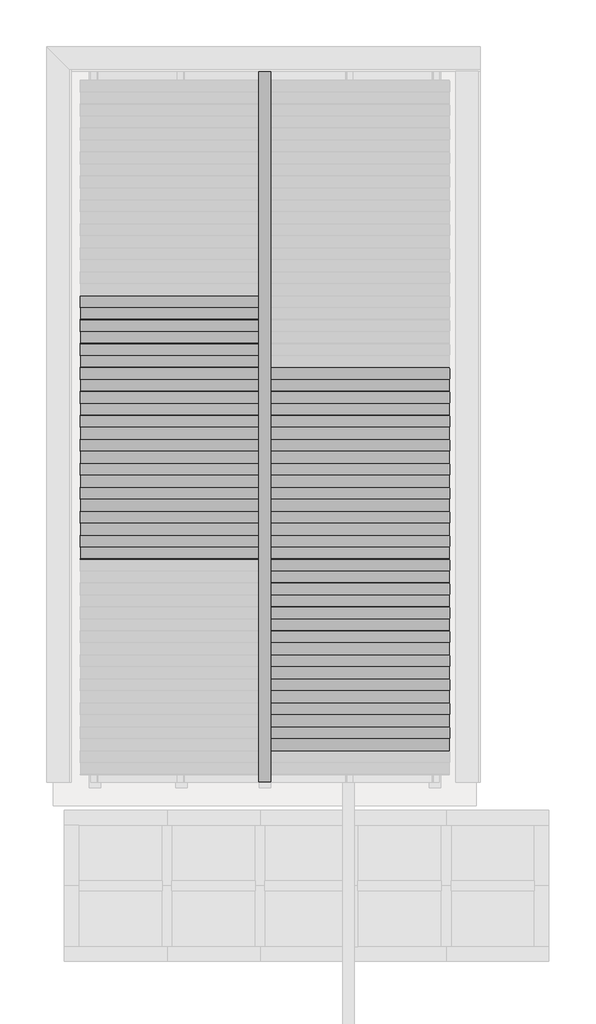
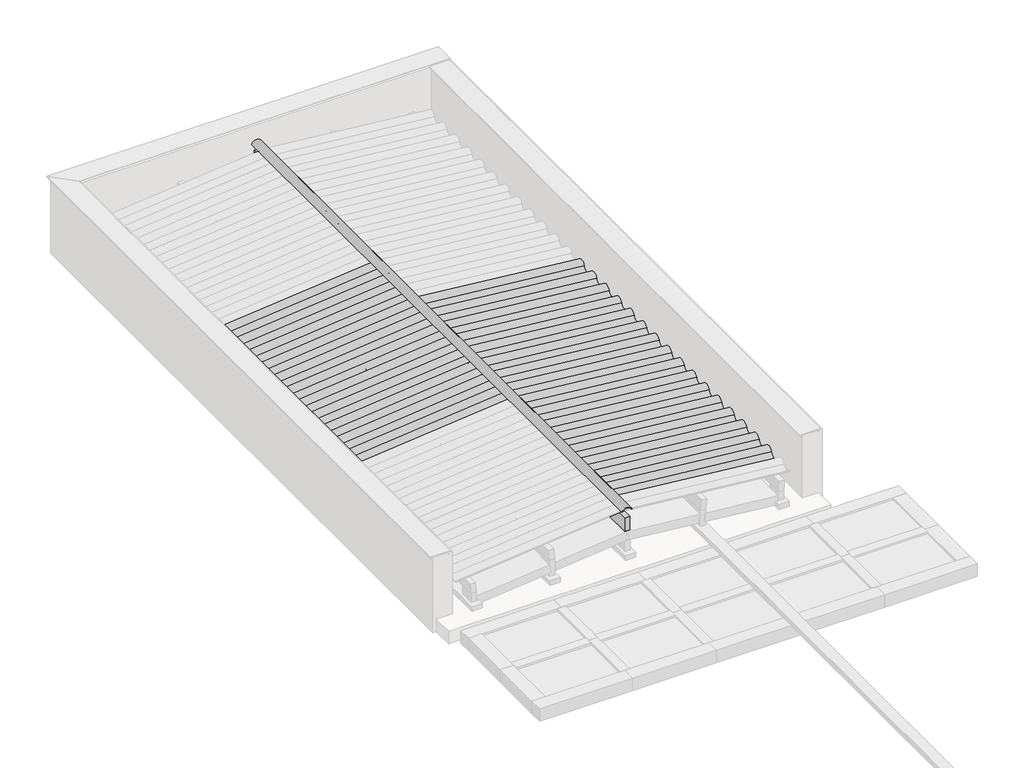
# One storey, part 2 of 3: 34 beams, 6 columns.
"""IFC4 building model written with IfcOpenShell, lengths in millimetres."""

import ifcopenshell
import ifcopenshell.guid

model = None  # the IFC model being written
_history = None  # IfcOwnerHistory: only IFC2X3 demands one
_inside = {}  # id of a spatial element -> (the spatial element, [elements in it])
_under = {}  # id of a project, library or spatial element -> (it, [spatial elements below it])
_declared = {}  # id of a project -> (the project, [libraries it declares])
_typed = {}  # id of a type object -> (the type object, [elements of that type])
_made_of = {}  # id of a material, layer set ... -> (it, [elements and type objects made of it])


def new_model(schema):
    """Start an empty IFC model of exactly this schema.

    Asked for "IFC4X3", IfcOpenShell would pick the latest addendum, in which some entities
    have other attributes; the version numbers below select the first issue.
    IFC2X3 requires an IfcOwnerHistory on every rooted entity: one is made here for all.
    """
    global model, _history
    if schema == "IFC4X3":
        model = ifcopenshell.file(schema_version=(4, 3, 0, 0))
    else:
        model = ifcopenshell.file(schema=schema)
    _inside.clear()
    _under.clear()
    _declared.clear()
    _typed.clear()
    _made_of.clear()
    _history = None
    if model.schema == "IFC2X3":
        org = make("IfcOrganization", Name="unknown")
        user = make(
            "IfcPersonAndOrganization",
            ThePerson=make("IfcPerson", FamilyName="unknown"),
            TheOrganization=org,
        )
        app = make(
            "IfcApplication",
            ApplicationDeveloper=org,
            Version="unknown",
            ApplicationFullName="unknown",
            ApplicationIdentifier="unknown",
        )
        _history = make(
            "IfcOwnerHistory",
            OwningUser=user,
            OwningApplication=app,
            ChangeAction="ADDED",
            CreationDate=0,
        )
    return model


def make(cls, **values):
    """One entity of the class cls with the attributes given. An attribute that is None is left unset."""
    return model.create_entity(
        cls, **{name: value for name, value in values.items() if value is not None}
    )


def rooted(cls, **values):
    """An entity with a GlobalId (a new one), such as an element, a storey or a relation."""
    return make(cls, GlobalId=ifcopenshell.guid.new(), OwnerHistory=_history, **values)


def si_unit(unit_type, name, prefix=None):
    """IfcSIUnit, for example si_unit("LENGTHUNIT", "METRE", prefix="MILLI")."""
    return make("IfcSIUnit", UnitType=unit_type, Prefix=prefix, Name=name)


def assignment(units):
    """IfcUnitAssignment: the units of a project."""
    return None if units is None else make("IfcUnitAssignment", Units=units)


def point(xyz):
    """IfcCartesianPoint."""
    return None if xyz is None else make("IfcCartesianPoint", Coordinates=xyz)


def direction(xyz):
    """IfcDirection."""
    return None if xyz is None else make("IfcDirection", DirectionRatios=xyz)


def frame(location, z_axis=None, x_axis=None):
    """IfcAxis2Placement3D, a coordinate frame: its origin and axes. An axis left out is left unset."""
    return make(
        "IfcAxis2Placement3D",
        Location=point(location),
        Axis=direction(z_axis),
        RefDirection=direction(x_axis),
    )


def frame_2d(location, x_axis=None):
    """IfcAxis2Placement2D, a coordinate frame in the plane: its origin and x axis."""
    return make(
        "IfcAxis2Placement2D", Location=point(location), RefDirection=direction(x_axis)
    )


def origin():
    """The frame at (0, 0, 0) with its axes left unset."""
    return frame((0.0, 0.0, 0.0))


def place(relative_to, where):
    """IfcLocalPlacement: puts the frame where relative to a parent placement (None: the world)."""
    return make(
        "IfcLocalPlacement", PlacementRelTo=relative_to, RelativePlacement=where
    )


def context(
    kind, dimensions, precision=None, world=None, true_north=None, identifier=None
):
    """IfcGeometricRepresentationContext, for example the 3D "Model" context."""
    return make(
        "IfcGeometricRepresentationContext",
        ContextIdentifier=identifier,
        ContextType=kind,
        CoordinateSpaceDimension=dimensions,
        Precision=precision,
        WorldCoordinateSystem=world,
        TrueNorth=true_north,
    )


def project(units=None, contexts=None):
    """IfcProject with its units and contexts."""
    return rooted(
        "IfcProject",
        Name="project",
        RepresentationContexts=contexts,
        UnitsInContext=assignment(units),
    )


def spatial(cls, under=None, at=None, **own):
    """A site, building, storey or space (cls), placed at a placement, below another one or the project."""
    s = rooted(cls, ObjectPlacement=at, **own)
    if under is not None:
        _under.setdefault(under.id(), (under, []))[1].append(s)
    return s


def polyline(points):
    """IfcPolyline through the points."""
    return make("IfcPolyline", Points=[point(p) for p in points])


def circle_curve(where, radius):
    """IfcCircle in the frame where."""
    return make("IfcCircle", Position=where, Radius=radius)


def trimmed(basis, trim1, trim2, sense, master):
    """IfcTrimmedCurve: the piece of a basis curve between two trims."""
    return make(
        "IfcTrimmedCurve",
        BasisCurve=basis,
        Trim1=trim1,
        Trim2=trim2,
        SenseAgreement=sense,
        MasterRepresentation=master,
    )


def segment(curve, same_sense, transition):
    """IfcCompositeCurveSegment."""
    return make(
        "IfcCompositeCurveSegment",
        Transition=transition,
        SameSense=same_sense,
        ParentCurve=curve,
    )


def composite_curve(segments, self_intersect=None):
    """IfcCompositeCurve: segments joined end to end."""
    return make("IfcCompositeCurve", Segments=segments, SelfIntersect=self_intersect)


def outline(outer, holes=None, kind="AREA"):
    """IfcArbitraryClosedProfileDef: a profile drawn as a closed curve; with holes, ...WithVoids."""
    if holes is None:
        return make("IfcArbitraryClosedProfileDef", ProfileType=kind, OuterCurve=outer)
    return make(
        "IfcArbitraryProfileDefWithVoids",
        ProfileType=kind,
        OuterCurve=outer,
        InnerCurves=holes,
    )


def extrude(swept, where, along, depth):
    """IfcExtrudedAreaSolid: the profile swept, set in the frame where, extruded along a direction by depth."""
    return make(
        "IfcExtrudedAreaSolid",
        SweptArea=swept,
        Position=where,
        ExtrudedDirection=direction(along),
        Depth=depth,
    )


def shape(context_of_items, identifier, shape_type, items):
    """IfcShapeRepresentation: the items that make up one representation, for example the "Body"."""
    return make(
        "IfcShapeRepresentation",
        ContextOfItems=context_of_items,
        RepresentationIdentifier=identifier,
        RepresentationType=shape_type,
        Items=items,
    )


def source(mapping_origin, context_of_items, identifier, shape_type, items):
    """IfcRepresentationMap: a shape defined once, which mapped items show again and again."""
    return make(
        "IfcRepresentationMap",
        MappingOrigin=mapping_origin,
        MappedRepresentation=shape(context_of_items, identifier, shape_type, items),
    )


def transform(
    local_origin,
    x_axis=None,
    y_axis=None,
    z_axis=None,
    scale=None,
    scale2=None,
    scale3=None,
    uniform=True,
):
    """IfcCartesianTransformationOperator3D, or its non-uniform kind. x_axis, y_axis, z_axis: its Axis1, 2, 3."""
    if uniform:
        return make(
            "IfcCartesianTransformationOperator3D",
            Axis1=direction(x_axis),
            Axis2=direction(y_axis),
            LocalOrigin=point(local_origin),
            Scale=scale,
            Axis3=direction(z_axis),
        )
    return make(
        "IfcCartesianTransformationOperator3DnonUniform",
        Axis1=direction(x_axis),
        Axis2=direction(y_axis),
        LocalOrigin=point(local_origin),
        Scale=scale,
        Axis3=direction(z_axis),
        Scale2=scale2,
        Scale3=scale3,
    )


def mapped(mapping_source, mapping_target):
    """IfcMappedItem: shows the shape of a source again, moved by a transform."""
    return make(
        "IfcMappedItem", MappingSource=mapping_source, MappingTarget=mapping_target
    )


def made_of(thing, what):
    """Note that an element or type object is made of a material, layer set ...; save() writes the relation."""
    if what is not None:
        _made_of.setdefault(what.id(), (what, []))[1].append(thing)
    return thing


def element(
    cls,
    number,
    at=None,
    inside=None,
    cuts=None,
    type_object=None,
    material=None,
    context=None,
    identifier="Body",
    shape_type=None,
    held_by="IfcProductDefinitionShape",
    body=None,
    shapes=None,
    **own,
):
    """One element of the class cls, such as IfcWall. Its Tag is "e" and its number.

    at: its placement. inside: the storey or other place that contains it. cuts: it is an
    opening in that element (IfcRelVoidsElement). A single representation is given by context,
    identifier, shape_type and body (its items); several are given by shapes. held_by: the class
    of the entity that holds the representations. save() writes the other relations.
    """
    e = rooted(cls, Tag="e%d" % number, ObjectPlacement=at, **own)
    if body is not None:
        shapes = [shape(context, identifier, shape_type, body)]
    if shapes is not None:
        e.Representation = make(held_by, Representations=shapes)
    if inside is not None:
        _inside.setdefault(inside.id(), (inside, []))[1].append(e)
    if cuts is not None:
        rooted(
            "IfcRelVoidsElement", RelatingBuildingElement=cuts, RelatedOpeningElement=e
        )
    if type_object is not None:
        _typed.setdefault(type_object.id(), (type_object, []))[1].append(e)
    return made_of(e, material)


def aggregate(whole, parts):
    """IfcRelAggregates: a whole, such as a stair, and the parts it consists of."""
    return rooted("IfcRelAggregates", RelatingObject=whole, RelatedObjects=parts)


def save(model, path):
    """Write the relations noted so far, then the file.

    IfcRelAggregates (storeys below a building ...), IfcRelContainedInSpatialStructure (elements
    in a storey), IfcRelDefinesByType, IfcRelAssociatesMaterial and IfcRelDeclares: one each for
    every whole, place, type object, material and project.
    """
    for whole, parts in _under.values():
        aggregate(whole, parts)
    for where, things in _inside.values():
        rooted(
            "IfcRelContainedInSpatialStructure",
            RelatedElements=things,
            RelatingStructure=where,
        )
    for kind, things in _typed.values():
        rooted("IfcRelDefinesByType", RelatedObjects=things, RelatingType=kind)
    for what, things in _made_of.values():
        rooted("IfcRelAssociatesMaterial", RelatedObjects=things, RelatingMaterial=what)
    for by, libraries in _declared.values():
        rooted("IfcRelDeclares", RelatingContext=by, RelatedDefinitions=libraries)
    model.write(path)


def cumeeira_telha_ondulada_fibrocimento_28917381(model_context):
    return source(origin(), model_context, "Body", "SweptSolid", [
        extrude(outline(composite_curve([segment(polyline([(58.3970135, 42.4437972), (53.9055884, 40.2467307)]), True, "CONTINUOUS"), segment(trimmed(circle_curve(frame_2d((-1.6029865, 13.0936483)), 61.7939461), [point((53.9055884, 40.2467307))], [point((-57.1115615, 40.2467307))], True, "CARTESIAN"), True, "CONTINUOUS"), segment(polyline([(-57.1115615, 40.2467307), (-61.6029865, 42.4437972)]), True, "CONTINUOUS"), segment(trimmed(circle_curve(frame_2d((-1.6029865, 13.0936483)), 66.7939461), [point((-61.6029865, 42.4437972))], [point((58.3970135, 42.4437972))], False, "CARTESIAN"), True, "CONTINUOUS")], self_intersect=False)), frame((-3626.5, 0.0, 0.0), z_axis=(1.0, 0.0, 0.0), x_axis=(0.0, 1.0, 0.0)), (0.0, 0.0, 1.0), 7253.0),
    ])


def viga_cumeeira_6x16cm_d80f05ee(model_context):
    return source(origin(), model_context, "Body", "SweptSolid", [
        extrude(outline(polyline([(3626.5, 30.0), (3626.5, -30.0), (-3626.5, -30.0), (-3626.5, 30.0), (3626.5, 30.0)])), frame((0.0, 0.0, -80.0), z_axis=(0.0, 0.0, 1.0), x_axis=(1.0, 0.0, 0.0)), (0.0, 0.0, 1.0), 160.0),
    ])


def column_1cffec27(model_context):
    return source(origin(), model_context, "Body", "SweptSolid", [
        extrude(outline(polyline([(30.0, 80.0), (30.0, -80.0), (-30.0, -80.0), (-30.0, 80.0), (30.0, 80.0)])), frame((0.0, 0.0, 3110.0), z_axis=(0.0, 0.0, 1.0), x_axis=(1.0, 0.0, 0.0)), (0.0, 0.0, 1.0), 238.0),
    ])


def column_35730ad5(model_context):
    return source(origin(), model_context, "Body", "SweptSolid", [
        extrude(outline(polyline([(30.0, 80.0), (30.0, -80.0), (-30.0, -80.0), (-30.0, 80.0), (30.0, 80.0)])), frame((0.0, 0.0, 3110.0), z_axis=(0.0, 0.0, 1.0), x_axis=(1.0, 0.0, 0.0)), (0.0, 0.0, 1.0), 197.9),
    ])


def column_00c463e4(model_context):
    return source(origin(), model_context, "Body", "SweptSolid", [
        extrude(outline(polyline([(30.0, 80.0), (30.0, -80.0), (-30.0, -80.0), (-30.0, 80.0), (30.0, 80.0)])), frame((0.0, 0.0, 3110.0), z_axis=(0.0, 0.0, 1.0), x_axis=(1.0, 0.0, 0.0)), (0.0, 0.0, 1.0), 109.8),
    ])


model = new_model("IFC4")

# Units and contexts
model_context = context("Model", 3, world=origin())
ifc_project = project(units=[si_unit("LENGTHUNIT", "METRE", prefix="MILLI")], contexts=[model_context])

# Site, building, storey
site = spatial("IfcSite", under=ifc_project)
building = spatial("IfcBuilding", under=site)
storey = spatial("IfcBuildingStorey", under=building, Name="COB. GARAGEM", Elevation=3050.0)

# Beams
placement = place(None, origin())
element("IfcBeam", 1, ObjectType="Madeira de lei : Berço 6x12cm", at=placement, inside=storey, context=model_context, shape_type="SweptSolid", body=[
    extrude(outline(polyline([(-9620.281307, 4423.9300153), (-9500.281307, 4423.9300153), (-9500.281307, 2423.9300153), (-9620.281307, 2423.9300153), (-9620.281307, 4423.9300153)])), frame((0.0, 0.0, 3050.0), z_axis=(0.0, 0.0, 1.0), x_axis=(1.0, 0.0, 0.0)), (0.0, 0.0, 1.0), 60.0),
])
element("IfcBeam", 2, ObjectType="Madeira de lei : Berço 6x12cm", at=placement, inside=storey, context=model_context, shape_type="SweptSolid", body=[
    extrude(outline(polyline([(-9620.281307, 2423.9300153), (-9500.281307, 2423.9300153), (-9500.281307, 423.9300153), (-9620.281307, 423.9300153), (-9620.281307, 2423.9300153)])), frame((0.0, 0.0, 3050.0), z_axis=(0.0, 0.0, 1.0), x_axis=(1.0, 0.0, 0.0)), (0.0, 0.0, 1.0), 60.0),
])
element("IfcBeam", 3, ObjectType="Madeira de lei : Berço 6x12cm", at=placement, inside=storey, context=model_context, shape_type="SweptSolid", body=[
    extrude(outline(polyline([(-8767.0824227, 4423.9300153), (-8647.0824227, 4423.9300153), (-8647.0824227, 2423.9300153), (-8767.0824227, 2423.9300153), (-8767.0824227, 4423.9300153)])), frame((0.0, 0.0, 3050.0), z_axis=(0.0, 0.0, 1.0), x_axis=(1.0, 0.0, 0.0)), (0.0, 0.0, 1.0), 60.0),
])
element("IfcBeam", 4, ObjectType="Madeira de lei : Berço 6x12cm", at=placement, inside=storey, context=model_context, shape_type="SweptSolid", body=[
    extrude(outline(polyline([(-10473.4801913, 4423.9300153), (-10353.4801913, 4423.9300153), (-10353.4801913, 2423.9300153), (-10473.4801913, 2423.9300153), (-10473.4801913, 4423.9300153)])), frame((0.0, 0.0, 3050.0), z_axis=(0.0, 0.0, 1.0), x_axis=(1.0, 0.0, 0.0)), (0.0, 0.0, 1.0), 60.0),
])
element("IfcBeam", 5, ObjectType="Madeira de lei : Berço 6x12cm", at=placement, inside=storey, context=model_context, shape_type="SweptSolid", body=[
    extrude(outline(polyline([(-11356.5301913, 4423.9300153), (-11236.5301913, 4423.9300153), (-11236.5301913, 2423.9300153), (-11356.5301913, 2423.9300153), (-11356.5301913, 4423.9300153)])), frame((0.0, 0.0, 3050.0), z_axis=(0.0, 0.0, 1.0), x_axis=(1.0, 0.0, 0.0)), (0.0, 0.0, 1.0), 60.0),
])
cumeeira_telha_ondulada_fibrocimento_shape = cumeeira_telha_ondulada_fibrocimento_28917381(model_context)
element("IfcBeam", 6, ObjectType="Cumeeira Telha Ondulada : Fibrocimento", at=placement, inside=storey, context=model_context, shape_type="MappedRepresentation", body=[
    mapped(cumeeira_telha_ondulada_fibrocimento_shape, transform((-9560.281307, 3455.9300153, 3545.9751229), x_axis=(0.0, -1.0, 0.0), y_axis=(1.0, 0.0, 0.0), z_axis=(0.0, 0.0, 1.0))),
])
element("IfcBeam", 7, ObjectType="Telha Ondulada : Fibrocimento", at=placement, inside=storey, context=model_context, shape_type="SweptSolid", body=[
    extrude(outline(composite_curve([segment(trimmed(circle_curve(frame_2d((-58.7002979, -53.2060538)), 66.7939461), [point((-29.350149, 6.7939462))], [point((-29.350149, -113.2060538))], False, "CARTESIAN"), True, "CONTINUOUS"), segment(polyline([(-29.350149, -113.2060538), (-31.5472155, -108.7146288)]), True, "CONTINUOUS"), segment(trimmed(circle_curve(frame_2d((-58.7002979, -53.2060538)), 61.7939461), [point((-31.5472155, -108.7146288))], [point((-31.5472155, 2.3025211))], True, "CARTESIAN"), True, "CONTINUOUS"), segment(trimmed(circle_curve(frame_2d((0.0, 66.7939462)), 71.7939461), [point((-31.5472155, 2.3025211))], [point((-31.5472155, 131.2853712))], False, "CARTESIAN"), True, "CONTINUOUS"), segment(polyline([(-31.5472155, 131.2853712), (-29.350149, 126.7939462)]), True, "CONTINUOUS"), segment(trimmed(circle_curve(frame_2d((0.0, 66.7939462)), 66.7939461), [point((-29.350149, 126.7939462))], [point((-29.350149, 6.7939462))], True, "CARTESIAN"), True, "CONTINUOUS")], self_intersect=False)), frame((-11446.918865, 2229.326948, 3394.3067746), z_axis=(0.9950371902099892, 0.0, 0.09950371902099919), x_axis=(-0.09950371902099919, 0.0, 0.9950371902099892)), (0.0, 0.0, 1.0), 1886.8678854),
])
element("IfcBeam", 8, ObjectType="Telha Ondulada : Fibrocimento", at=placement, inside=storey, context=model_context, shape_type="SweptSolid", body=[
    extrude(outline(composite_curve([segment(trimmed(circle_curve(frame_2d((-58.7002979, -53.2060538)), 66.7939461), [point((-29.350149, 6.7939462))], [point((-29.350149, -113.2060538))], False, "CARTESIAN"), True, "CONTINUOUS"), segment(polyline([(-29.350149, -113.2060538), (-31.5472155, -108.7146288)]), True, "CONTINUOUS"), segment(trimmed(circle_curve(frame_2d((-58.7002979, -53.2060538)), 61.7939461), [point((-31.5472155, -108.7146288))], [point((-31.5472155, 2.3025211))], True, "CARTESIAN"), True, "CONTINUOUS"), segment(trimmed(circle_curve(frame_2d((0.0, 66.7939462)), 71.7939461), [point((-31.5472155, 2.3025211))], [point((-31.5472155, 131.2853712))], False, "CARTESIAN"), True, "CONTINUOUS"), segment(polyline([(-31.5472155, 131.2853712), (-29.350149, 126.7939462)]), True, "CONTINUOUS"), segment(trimmed(circle_curve(frame_2d((0.0, 66.7939462)), 66.7939461), [point((-29.350149, 126.7939462))], [point((-29.350149, 6.7939462))], True, "CARTESIAN"), True, "CONTINUOUS")], self_intersect=False)), frame((-11446.918865, 2473.826948, 3394.3067746), z_axis=(0.9950371902099892, 0.0, 0.09950371902099932), x_axis=(-0.09950371902099932, 0.0, 0.9950371902099892)), (0.0, 0.0, 1.0), 1886.8678854),
])
element("IfcBeam", 9, ObjectType="Telha Ondulada : Fibrocimento", at=placement, inside=storey, context=model_context, shape_type="SweptSolid", body=[
    extrude(outline(composite_curve([segment(trimmed(circle_curve(frame_2d((-58.7002979, -53.2060538)), 66.7939461), [point((-29.350149, 6.7939462))], [point((-29.350149, -113.2060538))], False, "CARTESIAN"), True, "CONTINUOUS"), segment(polyline([(-29.350149, -113.2060538), (-31.5472155, -108.7146288)]), True, "CONTINUOUS"), segment(trimmed(circle_curve(frame_2d((-58.7002979, -53.2060538)), 61.7939461), [point((-31.5472155, -108.7146288))], [point((-31.5472155, 2.3025211))], True, "CARTESIAN"), True, "CONTINUOUS"), segment(trimmed(circle_curve(frame_2d((0.0, 66.7939462)), 71.7939461), [point((-31.5472155, 2.3025211))], [point((-31.5472155, 131.2853712))], False, "CARTESIAN"), True, "CONTINUOUS"), segment(polyline([(-31.5472155, 131.2853712), (-29.350149, 126.7939462)]), True, "CONTINUOUS"), segment(trimmed(circle_curve(frame_2d((0.0, 66.7939462)), 66.7939461), [point((-29.350149, 126.7939462))], [point((-29.350149, 6.7939462))], True, "CARTESIAN"), True, "CONTINUOUS")], self_intersect=False)), frame((-11446.918865, 2718.326948, 3394.3067746), z_axis=(0.9950371902099892, 0.0, 0.09950371902099937), x_axis=(-0.09950371902099937, 0.0, 0.9950371902099892)), (0.0, 0.0, 1.0), 1886.8678854),
])
element("IfcBeam", 10, ObjectType="Telha Ondulada : Fibrocimento", at=placement, inside=storey, context=model_context, shape_type="SweptSolid", body=[
    extrude(outline(composite_curve([segment(trimmed(circle_curve(frame_2d((-58.7002979, -53.2060538)), 66.7939461), [point((-29.350149, 6.7939462))], [point((-29.350149, -113.2060538))], False, "CARTESIAN"), True, "CONTINUOUS"), segment(polyline([(-29.350149, -113.2060538), (-31.5472155, -108.7146288)]), True, "CONTINUOUS"), segment(trimmed(circle_curve(frame_2d((-58.7002979, -53.2060538)), 61.7939461), [point((-31.5472155, -108.7146288))], [point((-31.5472155, 2.3025211))], True, "CARTESIAN"), True, "CONTINUOUS"), segment(trimmed(circle_curve(frame_2d((0.0, 66.7939462)), 71.7939461), [point((-31.5472155, 2.3025211))], [point((-31.5472155, 131.2853712))], False, "CARTESIAN"), True, "CONTINUOUS"), segment(polyline([(-31.5472155, 131.2853712), (-29.350149, 126.7939462)]), True, "CONTINUOUS"), segment(trimmed(circle_curve(frame_2d((0.0, 66.7939462)), 66.7939461), [point((-29.350149, 126.7939462))], [point((-29.350149, 6.7939462))], True, "CARTESIAN"), True, "CONTINUOUS")], self_intersect=False)), frame((-11446.918865, 2962.826948, 3394.3067746), z_axis=(0.9950371902099892, 0.0, 0.09950371902099943), x_axis=(-0.09950371902099943, 0.0, 0.9950371902099892)), (0.0, 0.0, 1.0), 1886.8678854),
])
element("IfcBeam", 11, ObjectType="Telha Ondulada : Fibrocimento", at=placement, inside=storey, context=model_context, shape_type="SweptSolid", body=[
    extrude(outline(composite_curve([segment(trimmed(circle_curve(frame_2d((-58.7002979, -53.2060538)), 66.7939461), [point((-29.350149, 6.7939462))], [point((-29.350149, -113.2060538))], False, "CARTESIAN"), True, "CONTINUOUS"), segment(polyline([(-29.350149, -113.2060538), (-31.5472155, -108.7146288)]), True, "CONTINUOUS"), segment(trimmed(circle_curve(frame_2d((-58.7002979, -53.2060538)), 61.7939461), [point((-31.5472155, -108.7146288))], [point((-31.5472155, 2.3025211))], True, "CARTESIAN"), True, "CONTINUOUS"), segment(trimmed(circle_curve(frame_2d((0.0, 66.7939462)), 71.7939461), [point((-31.5472155, 2.3025211))], [point((-31.5472155, 131.2853712))], False, "CARTESIAN"), True, "CONTINUOUS"), segment(polyline([(-31.5472155, 131.2853712), (-29.350149, 126.7939462)]), True, "CONTINUOUS"), segment(trimmed(circle_curve(frame_2d((0.0, 66.7939462)), 66.7939461), [point((-29.350149, 126.7939462))], [point((-29.350149, 6.7939462))], True, "CARTESIAN"), True, "CONTINUOUS")], self_intersect=False)), frame((-11446.918865, 3207.326948, 3394.3067746), z_axis=(0.9950371902099892, 0.0, 0.09950371902099954), x_axis=(-0.09950371902099954, 0.0, 0.9950371902099892)), (0.0, 0.0, 1.0), 1886.8678854),
])
element("IfcBeam", 12, ObjectType="Telha Ondulada : Fibrocimento", at=placement, inside=storey, context=model_context, shape_type="SweptSolid", body=[
    extrude(outline(composite_curve([segment(trimmed(circle_curve(frame_2d((-58.7002979, -53.2060538)), 66.7939461), [point((-29.350149, 6.7939462))], [point((-29.350149, -113.2060538))], False, "CARTESIAN"), True, "CONTINUOUS"), segment(polyline([(-29.350149, -113.2060538), (-31.5472155, -108.7146288)]), True, "CONTINUOUS"), segment(trimmed(circle_curve(frame_2d((-58.7002979, -53.2060538)), 61.7939461), [point((-31.5472155, -108.7146288))], [point((-31.5472155, 2.3025211))], True, "CARTESIAN"), True, "CONTINUOUS"), segment(trimmed(circle_curve(frame_2d((0.0, 66.7939462)), 71.7939461), [point((-31.5472155, 2.3025211))], [point((-31.5472155, 131.2853712))], False, "CARTESIAN"), True, "CONTINUOUS"), segment(polyline([(-31.5472155, 131.2853712), (-29.350149, 126.7939462)]), True, "CONTINUOUS"), segment(trimmed(circle_curve(frame_2d((0.0, 66.7939462)), 66.7939461), [point((-29.350149, 126.7939462))], [point((-29.350149, 6.7939462))], True, "CARTESIAN"), True, "CONTINUOUS")], self_intersect=False)), frame((-11446.918865, 3451.826948, 3394.3067746), z_axis=(0.9950371902099892, 0.0, 0.09950371902099937), x_axis=(-0.09950371902099937, 0.0, 0.9950371902099892)), (0.0, 0.0, 1.0), 1886.8678854),
])
element("IfcBeam", 13, ObjectType="Telha Ondulada : Fibrocimento", at=placement, inside=storey, context=model_context, shape_type="SweptSolid", body=[
    extrude(outline(composite_curve([segment(trimmed(circle_curve(frame_2d((-58.7002979, -53.2060538)), 66.7939461), [point((-29.350149, 6.7939462))], [point((-29.350149, -113.2060538))], False, "CARTESIAN"), True, "CONTINUOUS"), segment(polyline([(-29.350149, -113.2060538), (-31.5472155, -108.7146288)]), True, "CONTINUOUS"), segment(trimmed(circle_curve(frame_2d((-58.7002979, -53.2060538)), 61.7939461), [point((-31.5472155, -108.7146288))], [point((-31.5472155, 2.3025211))], True, "CARTESIAN"), True, "CONTINUOUS"), segment(trimmed(circle_curve(frame_2d((0.0, 66.7939462)), 71.7939461), [point((-31.5472155, 2.3025211))], [point((-31.5472155, 131.2853712))], False, "CARTESIAN"), True, "CONTINUOUS"), segment(polyline([(-31.5472155, 131.2853712), (-29.350149, 126.7939462)]), True, "CONTINUOUS"), segment(trimmed(circle_curve(frame_2d((0.0, 66.7939462)), 66.7939461), [point((-29.350149, 126.7939462))], [point((-29.350149, 6.7939462))], True, "CARTESIAN"), True, "CONTINUOUS")], self_intersect=False)), frame((-11446.918865, 3696.326948, 3394.3067746), z_axis=(0.9950371902099892, 0.0, 0.09950371902099914), x_axis=(-0.09950371902099914, 0.0, 0.9950371902099892)), (0.0, 0.0, 1.0), 1886.8678854),
])
element("IfcBeam", 14, ObjectType="Telha Ondulada : Fibrocimento", at=placement, inside=storey, context=model_context, shape_type="SweptSolid", body=[
    extrude(outline(composite_curve([segment(trimmed(circle_curve(frame_2d((-58.7002979, -53.2060538)), 66.7939461), [point((-29.350149, 6.7939462))], [point((-29.350149, -113.2060538))], False, "CARTESIAN"), True, "CONTINUOUS"), segment(polyline([(-29.350149, -113.2060538), (-31.5472155, -108.7146288)]), True, "CONTINUOUS"), segment(trimmed(circle_curve(frame_2d((-58.7002979, -53.2060538)), 61.7939461), [point((-31.5472155, -108.7146288))], [point((-31.5472155, 2.3025211))], True, "CARTESIAN"), True, "CONTINUOUS"), segment(trimmed(circle_curve(frame_2d((0.0, 66.7939462)), 71.7939461), [point((-31.5472155, 2.3025211))], [point((-31.5472155, 131.2853712))], False, "CARTESIAN"), True, "CONTINUOUS"), segment(polyline([(-31.5472155, 131.2853712), (-29.350149, 126.7939462)]), True, "CONTINUOUS"), segment(trimmed(circle_curve(frame_2d((0.0, 66.7939462)), 66.7939461), [point((-29.350149, 126.7939462))], [point((-29.350149, 6.7939462))], True, "CARTESIAN"), True, "CONTINUOUS")], self_intersect=False)), frame((-11446.918865, 3940.826948, 3394.3067746), z_axis=(0.9950371902099892, 0.0, 0.09950371902099948), x_axis=(-0.09950371902099948, 0.0, 0.9950371902099892)), (0.0, 0.0, 1.0), 1886.8678854),
])
element("IfcBeam", 15, ObjectType="Telha Ondulada : Fibrocimento", at=placement, inside=storey, context=model_context, shape_type="SweptSolid", body=[
    extrude(outline(composite_curve([segment(trimmed(circle_curve(frame_2d((-58.7002979, -53.2060538)), 66.7939461), [point((-29.350149, 6.7939462))], [point((-29.350149, -113.2060538))], False, "CARTESIAN"), True, "CONTINUOUS"), segment(polyline([(-29.350149, -113.2060538), (-31.5472155, -108.7146288)]), True, "CONTINUOUS"), segment(trimmed(circle_curve(frame_2d((-58.7002979, -53.2060538)), 61.7939461), [point((-31.5472155, -108.7146288))], [point((-31.5472155, 2.3025211))], True, "CARTESIAN"), True, "CONTINUOUS"), segment(trimmed(circle_curve(frame_2d((0.0, 66.7939462)), 71.7939461), [point((-31.5472155, 2.3025211))], [point((-31.5472155, 131.2853712))], False, "CARTESIAN"), True, "CONTINUOUS"), segment(polyline([(-31.5472155, 131.2853712), (-29.350149, 126.7939462)]), True, "CONTINUOUS"), segment(trimmed(circle_curve(frame_2d((0.0, 66.7939462)), 66.7939461), [point((-29.350149, 126.7939462))], [point((-29.350149, 6.7939462))], True, "CARTESIAN"), True, "CONTINUOUS")], self_intersect=False)), frame((-11446.918865, 4185.326948, 3394.3067746), z_axis=(0.9950371902099892, 0.0, 0.09950371902099932), x_axis=(-0.09950371902099932, 0.0, 0.9950371902099892)), (0.0, 0.0, 1.0), 1886.8678854),
])
element("IfcBeam", 16, ObjectType="Telha Ondulada : Fibrocimento", at=placement, inside=storey, context=model_context, shape_type="SweptSolid", body=[
    extrude(outline(composite_curve([segment(trimmed(circle_curve(frame_2d((-58.7002979, -53.2060538)), 66.7939461), [point((-29.350149, 6.7939462))], [point((-29.350149, -113.2060538))], False, "CARTESIAN"), True, "CONTINUOUS"), segment(polyline([(-29.350149, -113.2060538), (-31.5472155, -108.7146288)]), True, "CONTINUOUS"), segment(trimmed(circle_curve(frame_2d((-58.7002979, -53.2060538)), 61.7939461), [point((-31.5472155, -108.7146288))], [point((-31.5472155, 2.3025211))], True, "CARTESIAN"), True, "CONTINUOUS"), segment(trimmed(circle_curve(frame_2d((0.0, 66.7939462)), 71.7939461), [point((-31.5472155, 2.3025211))], [point((-31.5472155, 131.2853712))], False, "CARTESIAN"), True, "CONTINUOUS"), segment(polyline([(-31.5472155, 131.2853712), (-29.350149, 126.7939462)]), True, "CONTINUOUS"), segment(trimmed(circle_curve(frame_2d((0.0, 66.7939462)), 66.7939461), [point((-29.350149, 126.7939462))], [point((-29.350149, 6.7939462))], True, "CARTESIAN"), True, "CONTINUOUS")], self_intersect=False)), frame((-11446.918865, 4429.826948, 3394.3067746), z_axis=(0.9950371902099892, 0.0, 0.09950371902099943), x_axis=(-0.09950371902099943, 0.0, 0.9950371902099892)), (0.0, 0.0, 1.0), 1886.8678854),
])
element("IfcBeam", 17, ObjectType="Telha Ondulada : Fibrocimento", at=placement, inside=storey, context=model_context, shape_type="SweptSolid", body=[
    extrude(outline(composite_curve([segment(trimmed(circle_curve(frame_2d((-58.7002979, -53.2060538)), 66.7939461), [point((-29.350149, 6.7939462))], [point((-29.350149, -113.2060538))], False, "CARTESIAN"), True, "CONTINUOUS"), segment(polyline([(-29.350149, -113.2060538), (-31.5472155, -108.7146288)]), True, "CONTINUOUS"), segment(trimmed(circle_curve(frame_2d((-58.7002979, -53.2060538)), 61.7939461), [point((-31.5472155, -108.7146288))], [point((-31.5472155, 2.3025211))], True, "CARTESIAN"), True, "CONTINUOUS"), segment(trimmed(circle_curve(frame_2d((0.0, 66.7939462)), 71.7939461), [point((-31.5472155, 2.3025211))], [point((-31.5472155, 131.2853712))], False, "CARTESIAN"), True, "CONTINUOUS"), segment(polyline([(-31.5472155, 131.2853712), (-29.350149, 126.7939462)]), True, "CONTINUOUS"), segment(trimmed(circle_curve(frame_2d((0.0, 66.7939462)), 66.7939461), [point((-29.350149, 126.7939462))], [point((-29.350149, 6.7939462))], True, "CARTESIAN"), True, "CONTINUOUS")], self_intersect=False)), frame((-11446.918865, 4674.326948, 3394.3067746), z_axis=(0.9950371902099892, 0.0, 0.09950371902099943), x_axis=(-0.09950371902099943, 0.0, 0.9950371902099892)), (0.0, 0.0, 1.0), 1886.8678854),
])
element("IfcBeam", 18, ObjectType="Telha Ondulada : Fibrocimento", at=placement, inside=storey, context=model_context, shape_type="SweptSolid", body=[
    extrude(outline(composite_curve([segment(trimmed(circle_curve(frame_2d((0.0, 66.7939462)), 66.7939461), [point((29.350149, 6.7939462))], [point((29.350149, 126.7939462))], True, "CARTESIAN"), True, "CONTINUOUS"), segment(polyline([(29.350149, 126.7939462), (31.5472155, 131.2853712)]), True, "CONTINUOUS"), segment(trimmed(circle_curve(frame_2d((0.0, 66.7939462)), 71.7939461), [point((31.5472155, 131.2853712))], [point((31.5472155, 2.3025211))], False, "CARTESIAN"), True, "CONTINUOUS"), segment(trimmed(circle_curve(frame_2d((58.7002979, -53.2060538)), 61.7939461), [point((31.5472155, 2.3025211))], [point((31.5472155, -108.7146288))], True, "CARTESIAN"), True, "CONTINUOUS"), segment(polyline([(31.5472155, -108.7146288), (29.350149, -113.2060538)]), True, "CONTINUOUS"), segment(trimmed(circle_curve(frame_2d((58.7002979, -53.2060538)), 66.7939461), [point((29.350149, -113.2060538))], [point((29.350149, 6.7939462))], False, "CARTESIAN"), True, "CONTINUOUS")], self_intersect=False)), frame((-7673.6437489, 273.326948, 3394.3067746), z_axis=(-0.9950371902099892, 0.0, 0.09950371902099979), x_axis=(-0.09950371902099979, 0.0, -0.9950371902099892)), (0.0, 0.0, 1.0), 1886.8678854),
])
element("IfcBeam", 19, ObjectType="Telha Ondulada : Fibrocimento", at=placement, inside=storey, context=model_context, shape_type="SweptSolid", body=[
    extrude(outline(composite_curve([segment(trimmed(circle_curve(frame_2d((0.0, 66.7939462)), 66.7939461), [point((29.350149, 6.7939462))], [point((29.350149, 126.7939462))], True, "CARTESIAN"), True, "CONTINUOUS"), segment(polyline([(29.350149, 126.7939462), (31.5472155, 131.2853712)]), True, "CONTINUOUS"), segment(trimmed(circle_curve(frame_2d((0.0, 66.7939462)), 71.7939461), [point((31.5472155, 131.2853712))], [point((31.5472155, 2.3025211))], False, "CARTESIAN"), True, "CONTINUOUS"), segment(trimmed(circle_curve(frame_2d((58.7002979, -53.2060538)), 61.7939461), [point((31.5472155, 2.3025211))], [point((31.5472155, -108.7146288))], True, "CARTESIAN"), True, "CONTINUOUS"), segment(polyline([(31.5472155, -108.7146288), (29.350149, -113.2060538)]), True, "CONTINUOUS"), segment(trimmed(circle_curve(frame_2d((58.7002979, -53.2060538)), 66.7939461), [point((29.350149, -113.2060538))], [point((29.350149, 6.7939462))], False, "CARTESIAN"), True, "CONTINUOUS")], self_intersect=False)), frame((-7673.6437489, 517.826948, 3394.3067746), z_axis=(-0.9950371902099892, 0.0, 0.09950371902099979), x_axis=(-0.09950371902099979, 0.0, -0.9950371902099892)), (0.0, 0.0, 1.0), 1886.8678854),
])
element("IfcBeam", 20, ObjectType="Telha Ondulada : Fibrocimento", at=placement, inside=storey, context=model_context, shape_type="SweptSolid", body=[
    extrude(outline(composite_curve([segment(trimmed(circle_curve(frame_2d((0.0, 66.7939462)), 66.7939461), [point((29.350149, 6.7939462))], [point((29.350149, 126.7939462))], True, "CARTESIAN"), True, "CONTINUOUS"), segment(polyline([(29.350149, 126.7939462), (31.5472155, 131.2853712)]), True, "CONTINUOUS"), segment(trimmed(circle_curve(frame_2d((0.0, 66.7939462)), 71.7939461), [point((31.5472155, 131.2853712))], [point((31.5472155, 2.3025211))], False, "CARTESIAN"), True, "CONTINUOUS"), segment(trimmed(circle_curve(frame_2d((58.7002979, -53.2060538)), 61.7939461), [point((31.5472155, 2.3025211))], [point((31.5472155, -108.7146288))], True, "CARTESIAN"), True, "CONTINUOUS"), segment(polyline([(31.5472155, -108.7146288), (29.350149, -113.2060538)]), True, "CONTINUOUS"), segment(trimmed(circle_curve(frame_2d((58.7002979, -53.2060538)), 66.7939461), [point((29.350149, -113.2060538))], [point((29.350149, 6.7939462))], False, "CARTESIAN"), True, "CONTINUOUS")], self_intersect=False)), frame((-7673.6437489, 762.326948, 3394.3067746), z_axis=(-0.9950371902099892, 0.0, 0.09950371902099979), x_axis=(-0.09950371902099979, 0.0, -0.9950371902099892)), (0.0, 0.0, 1.0), 1886.8678854),
])
element("IfcBeam", 21, ObjectType="Telha Ondulada : Fibrocimento", at=placement, inside=storey, context=model_context, shape_type="SweptSolid", body=[
    extrude(outline(composite_curve([segment(trimmed(circle_curve(frame_2d((0.0, 66.7939462)), 66.7939461), [point((29.350149, 6.7939462))], [point((29.350149, 126.7939462))], True, "CARTESIAN"), True, "CONTINUOUS"), segment(polyline([(29.350149, 126.7939462), (31.5472155, 131.2853712)]), True, "CONTINUOUS"), segment(trimmed(circle_curve(frame_2d((0.0, 66.7939462)), 71.7939461), [point((31.5472155, 131.2853712))], [point((31.5472155, 2.3025211))], False, "CARTESIAN"), True, "CONTINUOUS"), segment(trimmed(circle_curve(frame_2d((58.7002979, -53.2060538)), 61.7939461), [point((31.5472155, 2.3025211))], [point((31.5472155, -108.7146288))], True, "CARTESIAN"), True, "CONTINUOUS"), segment(polyline([(31.5472155, -108.7146288), (29.350149, -113.2060538)]), True, "CONTINUOUS"), segment(trimmed(circle_curve(frame_2d((58.7002979, -53.2060538)), 66.7939461), [point((29.350149, -113.2060538))], [point((29.350149, 6.7939462))], False, "CARTESIAN"), True, "CONTINUOUS")], self_intersect=False)), frame((-7673.6437489, 1006.826948, 3394.3067746), z_axis=(-0.9950371902099892, 0.0, 0.09950371902099979), x_axis=(-0.09950371902099979, 0.0, -0.9950371902099892)), (0.0, 0.0, 1.0), 1886.8678854),
])
element("IfcBeam", 22, ObjectType="Telha Ondulada : Fibrocimento", at=placement, inside=storey, context=model_context, shape_type="SweptSolid", body=[
    extrude(outline(composite_curve([segment(trimmed(circle_curve(frame_2d((0.0, 66.7939462)), 66.7939461), [point((29.350149, 6.7939462))], [point((29.350149, 126.7939462))], True, "CARTESIAN"), True, "CONTINUOUS"), segment(polyline([(29.350149, 126.7939462), (31.5472155, 131.2853712)]), True, "CONTINUOUS"), segment(trimmed(circle_curve(frame_2d((0.0, 66.7939462)), 71.7939461), [point((31.5472155, 131.2853712))], [point((31.5472155, 2.3025211))], False, "CARTESIAN"), True, "CONTINUOUS"), segment(trimmed(circle_curve(frame_2d((58.7002979, -53.2060538)), 61.7939461), [point((31.5472155, 2.3025211))], [point((31.5472155, -108.7146288))], True, "CARTESIAN"), True, "CONTINUOUS"), segment(polyline([(31.5472155, -108.7146288), (29.350149, -113.2060538)]), True, "CONTINUOUS"), segment(trimmed(circle_curve(frame_2d((58.7002979, -53.2060538)), 66.7939461), [point((29.350149, -113.2060538))], [point((29.350149, 6.7939462))], False, "CARTESIAN"), True, "CONTINUOUS")], self_intersect=False)), frame((-7673.6437489, 1251.326948, 3394.3067746), z_axis=(-0.9950371902099892, 0.0, 0.09950371902099979), x_axis=(-0.09950371902099979, 0.0, -0.9950371902099892)), (0.0, 0.0, 1.0), 1886.8678854),
])
element("IfcBeam", 23, ObjectType="Telha Ondulada : Fibrocimento", at=placement, inside=storey, context=model_context, shape_type="SweptSolid", body=[
    extrude(outline(composite_curve([segment(trimmed(circle_curve(frame_2d((0.0, 66.7939462)), 66.7939461), [point((29.350149, 6.7939462))], [point((29.350149, 126.7939462))], True, "CARTESIAN"), True, "CONTINUOUS"), segment(polyline([(29.350149, 126.7939462), (31.5472155, 131.2853712)]), True, "CONTINUOUS"), segment(trimmed(circle_curve(frame_2d((0.0, 66.7939462)), 71.7939461), [point((31.5472155, 131.2853712))], [point((31.5472155, 2.3025211))], False, "CARTESIAN"), True, "CONTINUOUS"), segment(trimmed(circle_curve(frame_2d((58.7002979, -53.2060538)), 61.7939461), [point((31.5472155, 2.3025211))], [point((31.5472155, -108.7146288))], True, "CARTESIAN"), True, "CONTINUOUS"), segment(polyline([(31.5472155, -108.7146288), (29.350149, -113.2060538)]), True, "CONTINUOUS"), segment(trimmed(circle_curve(frame_2d((58.7002979, -53.2060538)), 66.7939461), [point((29.350149, -113.2060538))], [point((29.350149, 6.7939462))], False, "CARTESIAN"), True, "CONTINUOUS")], self_intersect=False)), frame((-7673.6437489, 1495.826948, 3394.3067746), z_axis=(-0.9950371902099892, 0.0, 0.09950371902099979), x_axis=(-0.09950371902099979, 0.0, -0.9950371902099892)), (0.0, 0.0, 1.0), 1886.8678854),
])
element("IfcBeam", 24, ObjectType="Telha Ondulada : Fibrocimento", at=placement, inside=storey, context=model_context, shape_type="SweptSolid", body=[
    extrude(outline(composite_curve([segment(trimmed(circle_curve(frame_2d((0.0, 66.7939462)), 66.7939461), [point((29.350149, 6.7939462))], [point((29.350149, 126.7939462))], True, "CARTESIAN"), True, "CONTINUOUS"), segment(polyline([(29.350149, 126.7939462), (31.5472155, 131.2853712)]), True, "CONTINUOUS"), segment(trimmed(circle_curve(frame_2d((0.0, 66.7939462)), 71.7939461), [point((31.5472155, 131.2853712))], [point((31.5472155, 2.3025211))], False, "CARTESIAN"), True, "CONTINUOUS"), segment(trimmed(circle_curve(frame_2d((58.7002979, -53.2060538)), 61.7939461), [point((31.5472155, 2.3025211))], [point((31.5472155, -108.7146288))], True, "CARTESIAN"), True, "CONTINUOUS"), segment(polyline([(31.5472155, -108.7146288), (29.350149, -113.2060538)]), True, "CONTINUOUS"), segment(trimmed(circle_curve(frame_2d((58.7002979, -53.2060538)), 66.7939461), [point((29.350149, -113.2060538))], [point((29.350149, 6.7939462))], False, "CARTESIAN"), True, "CONTINUOUS")], self_intersect=False)), frame((-7673.6437489, 1740.326948, 3394.3067746), z_axis=(-0.9950371902099892, 0.0, 0.09950371902099979), x_axis=(-0.09950371902099979, 0.0, -0.9950371902099892)), (0.0, 0.0, 1.0), 1886.8678854),
])
element("IfcBeam", 25, ObjectType="Telha Ondulada : Fibrocimento", at=placement, inside=storey, context=model_context, shape_type="SweptSolid", body=[
    extrude(outline(composite_curve([segment(trimmed(circle_curve(frame_2d((0.0, 66.7939462)), 66.7939461), [point((29.350149, 6.7939462))], [point((29.350149, 126.7939462))], True, "CARTESIAN"), True, "CONTINUOUS"), segment(polyline([(29.350149, 126.7939462), (31.5472155, 131.2853712)]), True, "CONTINUOUS"), segment(trimmed(circle_curve(frame_2d((0.0, 66.7939462)), 71.7939461), [point((31.5472155, 131.2853712))], [point((31.5472155, 2.3025211))], False, "CARTESIAN"), True, "CONTINUOUS"), segment(trimmed(circle_curve(frame_2d((58.7002979, -53.2060538)), 61.7939461), [point((31.5472155, 2.3025211))], [point((31.5472155, -108.7146288))], True, "CARTESIAN"), True, "CONTINUOUS"), segment(polyline([(31.5472155, -108.7146288), (29.350149, -113.2060538)]), True, "CONTINUOUS"), segment(trimmed(circle_curve(frame_2d((58.7002979, -53.2060538)), 66.7939461), [point((29.350149, -113.2060538))], [point((29.350149, 6.7939462))], False, "CARTESIAN"), True, "CONTINUOUS")], self_intersect=False)), frame((-7673.6437489, 1984.826948, 3394.3067746), z_axis=(-0.9950371902099892, 0.0, 0.09950371902099979), x_axis=(-0.09950371902099979, 0.0, -0.9950371902099892)), (0.0, 0.0, 1.0), 1886.8678854),
])
element("IfcBeam", 26, ObjectType="Telha Ondulada : Fibrocimento", at=placement, inside=storey, context=model_context, shape_type="SweptSolid", body=[
    extrude(outline(composite_curve([segment(trimmed(circle_curve(frame_2d((0.0, 66.7939462)), 66.7939461), [point((29.350149, 6.7939462))], [point((29.350149, 126.7939462))], True, "CARTESIAN"), True, "CONTINUOUS"), segment(polyline([(29.350149, 126.7939462), (31.5472155, 131.2853712)]), True, "CONTINUOUS"), segment(trimmed(circle_curve(frame_2d((0.0, 66.7939462)), 71.7939461), [point((31.5472155, 131.2853712))], [point((31.5472155, 2.3025211))], False, "CARTESIAN"), True, "CONTINUOUS"), segment(trimmed(circle_curve(frame_2d((58.7002979, -53.2060538)), 61.7939461), [point((31.5472155, 2.3025211))], [point((31.5472155, -108.7146288))], True, "CARTESIAN"), True, "CONTINUOUS"), segment(polyline([(31.5472155, -108.7146288), (29.350149, -113.2060538)]), True, "CONTINUOUS"), segment(trimmed(circle_curve(frame_2d((58.7002979, -53.2060538)), 66.7939461), [point((29.350149, -113.2060538))], [point((29.350149, 6.7939462))], False, "CARTESIAN"), True, "CONTINUOUS")], self_intersect=False)), frame((-7673.6437489, 2229.326948, 3394.3067746), z_axis=(-0.9950371902099892, 0.0, 0.09950371902099979), x_axis=(-0.09950371902099979, 0.0, -0.9950371902099892)), (0.0, 0.0, 1.0), 1886.8678854),
])
element("IfcBeam", 27, ObjectType="Telha Ondulada : Fibrocimento", at=placement, inside=storey, context=model_context, shape_type="SweptSolid", body=[
    extrude(outline(composite_curve([segment(trimmed(circle_curve(frame_2d((0.0, 66.7939462)), 66.7939461), [point((29.350149, 6.7939462))], [point((29.350149, 126.7939462))], True, "CARTESIAN"), True, "CONTINUOUS"), segment(polyline([(29.350149, 126.7939462), (31.5472155, 131.2853712)]), True, "CONTINUOUS"), segment(trimmed(circle_curve(frame_2d((0.0, 66.7939462)), 71.7939461), [point((31.5472155, 131.2853712))], [point((31.5472155, 2.3025211))], False, "CARTESIAN"), True, "CONTINUOUS"), segment(trimmed(circle_curve(frame_2d((58.7002979, -53.2060538)), 61.7939461), [point((31.5472155, 2.3025211))], [point((31.5472155, -108.7146288))], True, "CARTESIAN"), True, "CONTINUOUS"), segment(polyline([(31.5472155, -108.7146288), (29.350149, -113.2060538)]), True, "CONTINUOUS"), segment(trimmed(circle_curve(frame_2d((58.7002979, -53.2060538)), 66.7939461), [point((29.350149, -113.2060538))], [point((29.350149, 6.7939462))], False, "CARTESIAN"), True, "CONTINUOUS")], self_intersect=False)), frame((-7673.6437489, 2473.826948, 3394.3067746), z_axis=(-0.9950371902099892, 0.0, 0.09950371902099979), x_axis=(-0.09950371902099979, 0.0, -0.9950371902099892)), (0.0, 0.0, 1.0), 1886.8678854),
])
element("IfcBeam", 28, ObjectType="Telha Ondulada : Fibrocimento", at=placement, inside=storey, context=model_context, shape_type="SweptSolid", body=[
    extrude(outline(composite_curve([segment(trimmed(circle_curve(frame_2d((0.0, 66.7939462)), 66.7939461), [point((29.350149, 6.7939462))], [point((29.350149, 126.7939462))], True, "CARTESIAN"), True, "CONTINUOUS"), segment(polyline([(29.350149, 126.7939462), (31.5472155, 131.2853712)]), True, "CONTINUOUS"), segment(trimmed(circle_curve(frame_2d((0.0, 66.7939462)), 71.7939461), [point((31.5472155, 131.2853712))], [point((31.5472155, 2.3025211))], False, "CARTESIAN"), True, "CONTINUOUS"), segment(trimmed(circle_curve(frame_2d((58.7002979, -53.2060538)), 61.7939461), [point((31.5472155, 2.3025211))], [point((31.5472155, -108.7146288))], True, "CARTESIAN"), True, "CONTINUOUS"), segment(polyline([(31.5472155, -108.7146288), (29.350149, -113.2060538)]), True, "CONTINUOUS"), segment(trimmed(circle_curve(frame_2d((58.7002979, -53.2060538)), 66.7939461), [point((29.350149, -113.2060538))], [point((29.350149, 6.7939462))], False, "CARTESIAN"), True, "CONTINUOUS")], self_intersect=False)), frame((-7673.6437489, 2718.326948, 3394.3067746), z_axis=(-0.9950371902099892, 0.0, 0.09950371902099979), x_axis=(-0.09950371902099979, 0.0, -0.9950371902099892)), (0.0, 0.0, 1.0), 1886.8678854),
])
element("IfcBeam", 29, ObjectType="Telha Ondulada : Fibrocimento", at=placement, inside=storey, context=model_context, shape_type="SweptSolid", body=[
    extrude(outline(composite_curve([segment(trimmed(circle_curve(frame_2d((0.0, 66.7939462)), 66.7939461), [point((29.350149, 6.7939462))], [point((29.350149, 126.7939462))], True, "CARTESIAN"), True, "CONTINUOUS"), segment(polyline([(29.350149, 126.7939462), (31.5472155, 131.2853712)]), True, "CONTINUOUS"), segment(trimmed(circle_curve(frame_2d((0.0, 66.7939462)), 71.7939461), [point((31.5472155, 131.2853712))], [point((31.5472155, 2.3025211))], False, "CARTESIAN"), True, "CONTINUOUS"), segment(trimmed(circle_curve(frame_2d((58.7002979, -53.2060538)), 61.7939461), [point((31.5472155, 2.3025211))], [point((31.5472155, -108.7146288))], True, "CARTESIAN"), True, "CONTINUOUS"), segment(polyline([(31.5472155, -108.7146288), (29.350149, -113.2060538)]), True, "CONTINUOUS"), segment(trimmed(circle_curve(frame_2d((58.7002979, -53.2060538)), 66.7939461), [point((29.350149, -113.2060538))], [point((29.350149, 6.7939462))], False, "CARTESIAN"), True, "CONTINUOUS")], self_intersect=False)), frame((-7673.6437489, 2962.826948, 3394.3067746), z_axis=(-0.9950371902099892, 0.0, 0.09950371902099979), x_axis=(-0.09950371902099979, 0.0, -0.9950371902099892)), (0.0, 0.0, 1.0), 1886.8678854),
])
element("IfcBeam", 30, ObjectType="Telha Ondulada : Fibrocimento", at=placement, inside=storey, context=model_context, shape_type="SweptSolid", body=[
    extrude(outline(composite_curve([segment(trimmed(circle_curve(frame_2d((0.0, 66.7939462)), 66.7939461), [point((29.350149, 6.7939462))], [point((29.350149, 126.7939462))], True, "CARTESIAN"), True, "CONTINUOUS"), segment(polyline([(29.350149, 126.7939462), (31.5472155, 131.2853712)]), True, "CONTINUOUS"), segment(trimmed(circle_curve(frame_2d((0.0, 66.7939462)), 71.7939461), [point((31.5472155, 131.2853712))], [point((31.5472155, 2.3025211))], False, "CARTESIAN"), True, "CONTINUOUS"), segment(trimmed(circle_curve(frame_2d((58.7002979, -53.2060538)), 61.7939461), [point((31.5472155, 2.3025211))], [point((31.5472155, -108.7146288))], True, "CARTESIAN"), True, "CONTINUOUS"), segment(polyline([(31.5472155, -108.7146288), (29.350149, -113.2060538)]), True, "CONTINUOUS"), segment(trimmed(circle_curve(frame_2d((58.7002979, -53.2060538)), 66.7939461), [point((29.350149, -113.2060538))], [point((29.350149, 6.7939462))], False, "CARTESIAN"), True, "CONTINUOUS")], self_intersect=False)), frame((-7673.6437489, 3207.326948, 3394.3067746), z_axis=(-0.9950371902099892, 0.0, 0.09950371902099979), x_axis=(-0.09950371902099979, 0.0, -0.9950371902099892)), (0.0, 0.0, 1.0), 1886.8678854),
])
element("IfcBeam", 31, ObjectType="Telha Ondulada : Fibrocimento", at=placement, inside=storey, context=model_context, shape_type="SweptSolid", body=[
    extrude(outline(composite_curve([segment(trimmed(circle_curve(frame_2d((0.0, 66.7939462)), 66.7939461), [point((29.350149, 6.7939462))], [point((29.350149, 126.7939462))], True, "CARTESIAN"), True, "CONTINUOUS"), segment(polyline([(29.350149, 126.7939462), (31.5472155, 131.2853712)]), True, "CONTINUOUS"), segment(trimmed(circle_curve(frame_2d((0.0, 66.7939462)), 71.7939461), [point((31.5472155, 131.2853712))], [point((31.5472155, 2.3025211))], False, "CARTESIAN"), True, "CONTINUOUS"), segment(trimmed(circle_curve(frame_2d((58.7002979, -53.2060538)), 61.7939461), [point((31.5472155, 2.3025211))], [point((31.5472155, -108.7146288))], True, "CARTESIAN"), True, "CONTINUOUS"), segment(polyline([(31.5472155, -108.7146288), (29.350149, -113.2060538)]), True, "CONTINUOUS"), segment(trimmed(circle_curve(frame_2d((58.7002979, -53.2060538)), 66.7939461), [point((29.350149, -113.2060538))], [point((29.350149, 6.7939462))], False, "CARTESIAN"), True, "CONTINUOUS")], self_intersect=False)), frame((-7673.6437489, 3451.826948, 3394.3067746), z_axis=(-0.9950371902099892, 0.0, 0.09950371902099979), x_axis=(-0.09950371902099979, 0.0, -0.9950371902099892)), (0.0, 0.0, 1.0), 1886.8678854),
])
element("IfcBeam", 32, ObjectType="Telha Ondulada : Fibrocimento", at=placement, inside=storey, context=model_context, shape_type="SweptSolid", body=[
    extrude(outline(composite_curve([segment(trimmed(circle_curve(frame_2d((0.0, 66.7939462)), 66.7939461), [point((29.350149, 6.7939462))], [point((29.350149, 126.7939462))], True, "CARTESIAN"), True, "CONTINUOUS"), segment(polyline([(29.350149, 126.7939462), (31.5472155, 131.2853712)]), True, "CONTINUOUS"), segment(trimmed(circle_curve(frame_2d((0.0, 66.7939462)), 71.7939461), [point((31.5472155, 131.2853712))], [point((31.5472155, 2.3025211))], False, "CARTESIAN"), True, "CONTINUOUS"), segment(trimmed(circle_curve(frame_2d((58.7002979, -53.2060538)), 61.7939461), [point((31.5472155, 2.3025211))], [point((31.5472155, -108.7146288))], True, "CARTESIAN"), True, "CONTINUOUS"), segment(polyline([(31.5472155, -108.7146288), (29.350149, -113.2060538)]), True, "CONTINUOUS"), segment(trimmed(circle_curve(frame_2d((58.7002979, -53.2060538)), 66.7939461), [point((29.350149, -113.2060538))], [point((29.350149, 6.7939462))], False, "CARTESIAN"), True, "CONTINUOUS")], self_intersect=False)), frame((-7673.6437489, 3696.326948, 3394.3067746), z_axis=(-0.9950371902099892, 0.0, 0.09950371902099979), x_axis=(-0.09950371902099979, 0.0, -0.9950371902099892)), (0.0, 0.0, 1.0), 1886.8678854),
])
element("IfcBeam", 33, ObjectType="Telha Ondulada : Fibrocimento", at=placement, inside=storey, context=model_context, shape_type="SweptSolid", body=[
    extrude(outline(composite_curve([segment(trimmed(circle_curve(frame_2d((0.0, 66.7939462)), 66.7939461), [point((29.350149, 6.7939462))], [point((29.350149, 126.7939462))], True, "CARTESIAN"), True, "CONTINUOUS"), segment(polyline([(29.350149, 126.7939462), (31.5472155, 131.2853712)]), True, "CONTINUOUS"), segment(trimmed(circle_curve(frame_2d((0.0, 66.7939462)), 71.7939461), [point((31.5472155, 131.2853712))], [point((31.5472155, 2.3025211))], False, "CARTESIAN"), True, "CONTINUOUS"), segment(trimmed(circle_curve(frame_2d((58.7002979, -53.2060538)), 61.7939461), [point((31.5472155, 2.3025211))], [point((31.5472155, -108.7146288))], True, "CARTESIAN"), True, "CONTINUOUS"), segment(polyline([(31.5472155, -108.7146288), (29.350149, -113.2060538)]), True, "CONTINUOUS"), segment(trimmed(circle_curve(frame_2d((58.7002979, -53.2060538)), 66.7939461), [point((29.350149, -113.2060538))], [point((29.350149, 6.7939462))], False, "CARTESIAN"), True, "CONTINUOUS")], self_intersect=False)), frame((-7673.6437489, 3940.826948, 3394.3067746), z_axis=(-0.9950371902099892, 0.0, 0.09950371902099979), x_axis=(-0.09950371902099979, 0.0, -0.9950371902099892)), (0.0, 0.0, 1.0), 1886.8678854),
])
viga_cumeeira_6x16cm_shape = viga_cumeeira_6x16cm_d80f05ee(model_context)
element("IfcBeam", 34, ObjectType="Madeira de lei : Viga Cumeeira 6x16cm", at=placement, inside=storey, context=model_context, shape_type="MappedRepresentation", body=[
    mapped(viga_cumeeira_6x16cm_shape, transform((-9560.281307, 3455.9300153, 3427.8), x_axis=(0.0, -1.0, 0.0), y_axis=(1.0, 0.0, 0.0), z_axis=(0.0, 0.0, 1.0))),
])

# Columns
column_shape = column_1cffec27(model_context)
element("IfcColumn", 35, ObjectType="Madeira de lei-Coluna : Pontalete 6X16cm", at=placement, inside=storey, context=model_context, shape_type="MappedRepresentation", body=[
    mapped(column_shape, transform((-9560.281307, 3423.9300153, 0.0), x_axis=(1.0, 0.0, 0.0), y_axis=(0.0, 1.0, 0.0), z_axis=(0.0, 0.0, 1.0))),
])
element("IfcColumn", 36, ObjectType="Madeira de lei-Coluna : Pontalete 6X16cm", at=placement, inside=storey, context=model_context, shape_type="MappedRepresentation", body=[
    mapped(column_shape, transform((-9560.281307, 1423.9300153, 0.0), x_axis=(1.0, 0.0, 0.0), y_axis=(0.0, 1.0, 0.0), z_axis=(0.0, 0.0, 1.0))),
])
column_2_shape = column_35730ad5(model_context)
element("IfcColumn", 37, ObjectType="Madeira de lei-Coluna : Pontalete 6X16cm", at=placement, inside=storey, context=model_context, shape_type="MappedRepresentation", body=[
    mapped(column_2_shape, transform((-8707.0824227, 3423.9300153, 0.0), x_axis=(1.0, 0.0, 0.0), y_axis=(0.0, 1.0, 0.0), z_axis=(0.0, 0.0, 1.0))),
])
element("IfcColumn", 38, ObjectType="Madeira de lei-Coluna : Pontalete 6X16cm", at=placement, inside=storey, context=model_context, shape_type="MappedRepresentation", body=[
    mapped(column_2_shape, transform((-8707.0824227, 1423.9300153, 0.0), x_axis=(1.0, 0.0, 0.0), y_axis=(0.0, 1.0, 0.0), z_axis=(0.0, 0.0, 1.0))),
])
element("IfcColumn", 39, ObjectType="Madeira de lei-Coluna : Pontalete 6X16cm", at=placement, inside=storey, context=model_context, shape_type="MappedRepresentation", body=[
    mapped(column_2_shape, transform((-10413.4801913, 3423.9300153, 0.0), x_axis=(1.0, 0.0, 0.0), y_axis=(0.0, 1.0, 0.0), z_axis=(0.0, 0.0, 1.0))),
])
column_3_shape = column_00c463e4(model_context)
element("IfcColumn", 40, ObjectType="Madeira de lei-Coluna : Pontalete 6X16cm", at=placement, inside=storey, context=model_context, shape_type="MappedRepresentation", body=[
    mapped(column_3_shape, transform((-11296.5301913, 3423.9300153, 0.0), x_axis=(1.0, 0.0, 0.0), y_axis=(0.0, 1.0, 0.0), z_axis=(0.0, 0.0, 1.0))),
])

save(model, "model.ifc")

# Revit data of these elements
# Type "Madeira de lei : Berço 6x12cm"
#   A = 0.02 m²
#   Length [instance default] = 1.524 m
#   b = 0.06 m
#   d = 0.12 m
#   Structural Material [instance default] = none
#   Assembly Code = ""
# Type "Cumeeira Telha Ondulada : Fibrocimento"
#   Cost = 5
#   Length [instance default] = 1.524 m
#   b = 0.07 m
#   h = 0.16 m
#   Structural Material = .TELHA DE FIBROCIMENTO
#   Assembly Code = ""
# Type "Telha Ondulada : Fibrocimento"
#   Description = "TELHA ONDULADA FIBROCIMENTO"
#   Cost = 5
#   Length [instance default] = 1.524 m
#   b = 0.07 m
#   h = 0.16 m
#   Structural Material = .TELHA DE FIBROCIMENTO
#   Assembly Code = ""
# Type "Madeira de lei : Viga Cumeeira 6x16cm"
#   A = 0.02 m²
#   Length [instance default] = 1.524 m
#   b = 0.06 m
#   d = 0.16 m
#   Structural Material [instance default] = none
#   Assembly Code = ""
# Type "Madeira de lei-Coluna : Pontalete 6X16cm"
#   A = 0.01952 m²
#   b = 0.06 m
#   d = 0.16 m
#   Structural Material [instance default] = none
#   Assembly Code = ""
# Elements 1, 2, 3, 4, 5 (IfcBeam, "Madeira de lei : Berço 6x12cm")
#   Comments = ""
#   Uso = "TELHADOS ESTRUTURAS"
#   Compr Cmcl = 6.00 m
#   Structural Material = .MADEIRAMENTO
#   Phase Created = CC_AP
#   Materials on its faces: ".MADEIRAMENTO"
# Element 6 (IfcBeam, "Cumeeira Telha Ondulada : Fibrocimento")
#   Comments = ""
#   Uso = "TELHADOS TELHAS"
#   Phase Created = CC_AP
#   Materials on its faces: ".TELHA DE FIBROCIMENTO"
# Elements 7, 8, 9, 10, 11, 12, 13, 14, 15, 16, 17, 18, 19, 20, 21, 22, 23, 24, 25, 26, 27, 28, 29, 30, 31, 32, 33 (IfcBeam, "Telha Ondulada : Fibrocimento")
#   Uso = "TELHADOS TELHAS"
#   Phase Created = CC_AP
#   Materials on its faces: ".TELHA DE FIBROCIMENTO"
# Element 34 (IfcBeam, "Madeira de lei : Viga Cumeeira 6x16cm")
#   Comments = ""
#   Uso = "TELHADOS MADEIRAMENTO"
#   Compr Cmcl = 7.50 m
#   Structural Material = .MADEIRAMENTO
#   Phase Created = CC_AP
#   Materials on its faces: ".MADEIRAMENTO"
# Elements 35, 36, 37, 38, 39, 40 (IfcColumn, "Madeira de lei-Coluna : Pontalete 6X16cm")
#   Comments = ""
#   Uso = "TELHADOS ESTRUTURAS"
#   Compr Cmcl = 2.00 m
#   Structural Material = .MADEIRAMENTO
#   Phase Created = CC_AP
#   Materials on its faces: ".MADEIRAMENTO"
# Materials
#   ".TELHA DE FIBROCIMENTO": class "CC_TELHADO", colour RGB 77 77 76, transparency 0, Description = "TELHA ONDULADA FIBROCIMENTO", Cost = 0
#   ".MADEIRAMENTO": class ".CC_MADEIRAS", colour RGB 212 179 113, transparency 0, Cost = 0
# Room, not placed, phase "CC_AP", upper offset 0.00 m, lower offset 0.00 m
#   Number = "31"
#   Name = "Room"
# Room, not placed, phase "CC_AP", upper offset 0.00 m, lower offset 0.00 m
#   Number = "34"
#   Name = "Room"
